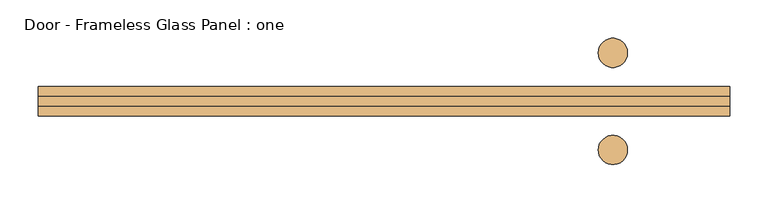
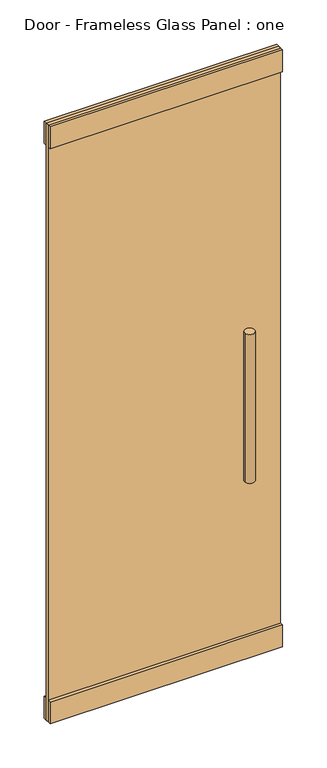
"""IFC4 building model written with IfcOpenShell, lengths in millimetres: door geometry, Door - Frameless Glass Panel : one."""

import ifcopenshell
import ifcopenshell.guid

model = None  # the IFC model being written
_history = None  # IfcOwnerHistory: only IFC2X3 demands one
_inside = {}  # id of a spatial element -> (the spatial element, [elements in it])
_under = {}  # id of a project, library or spatial element -> (it, [spatial elements below it])
_declared = {}  # id of a project -> (the project, [libraries it declares])
_typed = {}  # id of a type object -> (the type object, [elements of that type])
_made_of = {}  # id of a material, layer set ... -> (it, [elements and type objects made of it])


def new_model(schema):
    """Start an empty IFC model of exactly this schema.

    Asked for "IFC4X3", IfcOpenShell would pick the latest addendum, in which some entities
    have other attributes; the version numbers below select the first issue.
    IFC2X3 requires an IfcOwnerHistory on every rooted entity: one is made here for all.
    """
    global model, _history
    if schema == "IFC4X3":
        model = ifcopenshell.file(schema_version=(4, 3, 0, 0))
    else:
        model = ifcopenshell.file(schema=schema)
    _inside.clear()
    _under.clear()
    _declared.clear()
    _typed.clear()
    _made_of.clear()
    _history = None
    if model.schema == "IFC2X3":
        org = make("IfcOrganization", Name="unknown")
        user = make(
            "IfcPersonAndOrganization",
            ThePerson=make("IfcPerson", FamilyName="unknown"),
            TheOrganization=org,
        )
        app = make(
            "IfcApplication",
            ApplicationDeveloper=org,
            Version="unknown",
            ApplicationFullName="unknown",
            ApplicationIdentifier="unknown",
        )
        _history = make(
            "IfcOwnerHistory",
            OwningUser=user,
            OwningApplication=app,
            ChangeAction="ADDED",
            CreationDate=0,
        )
    return model


def make(cls, **values):
    """One entity of the class cls with the attributes given. An attribute that is None is left unset."""
    return model.create_entity(
        cls, **{name: value for name, value in values.items() if value is not None}
    )


def rooted(cls, **values):
    """An entity with a GlobalId (a new one), such as an element, a storey or a relation."""
    return make(cls, GlobalId=ifcopenshell.guid.new(), OwnerHistory=_history, **values)


def si_unit(unit_type, name, prefix=None):
    """IfcSIUnit, for example si_unit("LENGTHUNIT", "METRE", prefix="MILLI")."""
    return make("IfcSIUnit", UnitType=unit_type, Prefix=prefix, Name=name)


def assignment(units):
    """IfcUnitAssignment: the units of a project."""
    return None if units is None else make("IfcUnitAssignment", Units=units)


def point(xyz):
    """IfcCartesianPoint."""
    return None if xyz is None else make("IfcCartesianPoint", Coordinates=xyz)


def direction(xyz):
    """IfcDirection."""
    return None if xyz is None else make("IfcDirection", DirectionRatios=xyz)


def frame(location, z_axis=None, x_axis=None):
    """IfcAxis2Placement3D, a coordinate frame: its origin and axes. An axis left out is left unset."""
    return make(
        "IfcAxis2Placement3D",
        Location=point(location),
        Axis=direction(z_axis),
        RefDirection=direction(x_axis),
    )


def frame_2d(location, x_axis=None):
    """IfcAxis2Placement2D, a coordinate frame in the plane: its origin and x axis."""
    return make(
        "IfcAxis2Placement2D", Location=point(location), RefDirection=direction(x_axis)
    )


def origin():
    """The frame at (0, 0, 0) with its axes left unset."""
    return frame((0.0, 0.0, 0.0))


def origin_with_axes():
    """The frame at (0, 0, 0) with the z axis (0, 0, 1) and the x axis (1, 0, 0) written out."""
    return frame((0.0, 0.0, 0.0), z_axis=(0.0, 0.0, 1.0), x_axis=(1.0, 0.0, 0.0))


def place(relative_to, where):
    """IfcLocalPlacement: puts the frame where relative to a parent placement (None: the world)."""
    return make(
        "IfcLocalPlacement", PlacementRelTo=relative_to, RelativePlacement=where
    )


def context(
    kind, dimensions, precision=None, world=None, true_north=None, identifier=None
):
    """IfcGeometricRepresentationContext, for example the 3D "Model" context."""
    return make(
        "IfcGeometricRepresentationContext",
        ContextIdentifier=identifier,
        ContextType=kind,
        CoordinateSpaceDimension=dimensions,
        Precision=precision,
        WorldCoordinateSystem=world,
        TrueNorth=true_north,
    )


def project(units=None, contexts=None):
    """IfcProject with its units and contexts."""
    return rooted(
        "IfcProject",
        Name="project",
        RepresentationContexts=contexts,
        UnitsInContext=assignment(units),
    )


def spatial(cls, under=None, at=None, **own):
    """A site, building, storey or space (cls), placed at a placement, below another one or the project."""
    s = rooted(cls, ObjectPlacement=at, **own)
    if under is not None:
        _under.setdefault(under.id(), (under, []))[1].append(s)
    return s


def polyline(points):
    """IfcPolyline through the points."""
    return make("IfcPolyline", Points=[point(p) for p in points])


def circle_curve(where, radius):
    """IfcCircle in the frame where."""
    return make("IfcCircle", Position=where, Radius=radius)


def trimmed(basis, trim1, trim2, sense, master):
    """IfcTrimmedCurve: the piece of a basis curve between two trims."""
    return make(
        "IfcTrimmedCurve",
        BasisCurve=basis,
        Trim1=trim1,
        Trim2=trim2,
        SenseAgreement=sense,
        MasterRepresentation=master,
    )


def segment(curve, same_sense, transition):
    """IfcCompositeCurveSegment."""
    return make(
        "IfcCompositeCurveSegment",
        Transition=transition,
        SameSense=same_sense,
        ParentCurve=curve,
    )


def composite_curve(segments, self_intersect=None):
    """IfcCompositeCurve: segments joined end to end."""
    return make("IfcCompositeCurve", Segments=segments, SelfIntersect=self_intersect)


def outline(outer, holes=None, kind="AREA"):
    """IfcArbitraryClosedProfileDef: a profile drawn as a closed curve; with holes, ...WithVoids."""
    if holes is None:
        return make("IfcArbitraryClosedProfileDef", ProfileType=kind, OuterCurve=outer)
    return make(
        "IfcArbitraryProfileDefWithVoids",
        ProfileType=kind,
        OuterCurve=outer,
        InnerCurves=holes,
    )


def extrude(swept, where, along, depth):
    """IfcExtrudedAreaSolid: the profile swept, set in the frame where, extruded along a direction by depth."""
    return make(
        "IfcExtrudedAreaSolid",
        SweptArea=swept,
        Position=where,
        ExtrudedDirection=direction(along),
        Depth=depth,
    )


def shape(context_of_items, identifier, shape_type, items):
    """IfcShapeRepresentation: the items that make up one representation, for example the "Body"."""
    return make(
        "IfcShapeRepresentation",
        ContextOfItems=context_of_items,
        RepresentationIdentifier=identifier,
        RepresentationType=shape_type,
        Items=items,
    )


def source(mapping_origin, context_of_items, identifier, shape_type, items):
    """IfcRepresentationMap: a shape defined once, which mapped items show again and again."""
    return make(
        "IfcRepresentationMap",
        MappingOrigin=mapping_origin,
        MappedRepresentation=shape(context_of_items, identifier, shape_type, items),
    )


def transform(
    local_origin,
    x_axis=None,
    y_axis=None,
    z_axis=None,
    scale=None,
    scale2=None,
    scale3=None,
    uniform=True,
):
    """IfcCartesianTransformationOperator3D, or its non-uniform kind. x_axis, y_axis, z_axis: its Axis1, 2, 3."""
    if uniform:
        return make(
            "IfcCartesianTransformationOperator3D",
            Axis1=direction(x_axis),
            Axis2=direction(y_axis),
            LocalOrigin=point(local_origin),
            Scale=scale,
            Axis3=direction(z_axis),
        )
    return make(
        "IfcCartesianTransformationOperator3DnonUniform",
        Axis1=direction(x_axis),
        Axis2=direction(y_axis),
        LocalOrigin=point(local_origin),
        Scale=scale,
        Axis3=direction(z_axis),
        Scale2=scale2,
        Scale3=scale3,
    )


def mapped(mapping_source, mapping_target):
    """IfcMappedItem: shows the shape of a source again, moved by a transform."""
    return make(
        "IfcMappedItem", MappingSource=mapping_source, MappingTarget=mapping_target
    )


def made_of(thing, what):
    """Note that an element or type object is made of a material, layer set ...; save() writes the relation."""
    if what is not None:
        _made_of.setdefault(what.id(), (what, []))[1].append(thing)
    return thing


def element(
    cls,
    number,
    at=None,
    inside=None,
    cuts=None,
    type_object=None,
    material=None,
    context=None,
    identifier="Body",
    shape_type=None,
    held_by="IfcProductDefinitionShape",
    body=None,
    shapes=None,
    **own,
):
    """One element of the class cls, such as IfcWall. Its Tag is "e" and its number.

    at: its placement. inside: the storey or other place that contains it. cuts: it is an
    opening in that element (IfcRelVoidsElement). A single representation is given by context,
    identifier, shape_type and body (its items); several are given by shapes. held_by: the class
    of the entity that holds the representations. save() writes the other relations.
    """
    e = rooted(cls, Tag="e%d" % number, ObjectPlacement=at, **own)
    if body is not None:
        shapes = [shape(context, identifier, shape_type, body)]
    if shapes is not None:
        e.Representation = make(held_by, Representations=shapes)
    if inside is not None:
        _inside.setdefault(inside.id(), (inside, []))[1].append(e)
    if cuts is not None:
        rooted(
            "IfcRelVoidsElement", RelatingBuildingElement=cuts, RelatedOpeningElement=e
        )
    if type_object is not None:
        _typed.setdefault(type_object.id(), (type_object, []))[1].append(e)
    return made_of(e, material)


def aggregate(whole, parts):
    """IfcRelAggregates: a whole, such as a stair, and the parts it consists of."""
    return rooted("IfcRelAggregates", RelatingObject=whole, RelatedObjects=parts)


def save(model, path):
    """Write the relations noted so far, then the file.

    IfcRelAggregates (storeys below a building ...), IfcRelContainedInSpatialStructure (elements
    in a storey), IfcRelDefinesByType, IfcRelAssociatesMaterial and IfcRelDeclares: one each for
    every whole, place, type object, material and project.
    """
    for whole, parts in _under.values():
        aggregate(whole, parts)
    for where, things in _inside.values():
        rooted(
            "IfcRelContainedInSpatialStructure",
            RelatedElements=things,
            RelatingStructure=where,
        )
    for kind, things in _typed.values():
        rooted("IfcRelDefinesByType", RelatedObjects=things, RelatingType=kind)
    for what, things in _made_of.values():
        rooted("IfcRelAssociatesMaterial", RelatedObjects=things, RelatingMaterial=what)
    for by, libraries in _declared.values():
        rooted("IfcRelDeclares", RelatingContext=by, RelatedDefinitions=libraries)
    model.write(path)


def door_frameless_glass_panel_one_304fad4e(model_context):
    return source(origin(), model_context, "Body", "SweptSolid", [
        extrude(outline(composite_curve([segment(trimmed(circle_curve(frame_2d((298.45, -63.5)), 19.05), [point((279.4, -63.5))], [point((317.5, -63.5))], False, "CARTESIAN"), True, "CONTINUOUS"), segment(trimmed(circle_curve(frame_2d((298.45, -63.5)), 19.05), [point((317.5, -63.5))], [point((279.4, -63.5))], False, "CARTESIAN"), True, "CONTINUOUS")], self_intersect=False)), frame((0.0, 0.0, 762.0), z_axis=(0.0, 0.0, 1.0), x_axis=(1.0, 0.0, 0.0)), (0.0, 0.0, 1.0), 609.6),
        extrude(outline(composite_curve([segment(trimmed(circle_curve(frame_2d((298.45, 63.5)), 19.05), [point((279.4, 63.5))], [point((317.5, 63.5))], False, "CARTESIAN"), True, "CONTINUOUS"), segment(trimmed(circle_curve(frame_2d((298.45, 63.5)), 19.05), [point((317.5, 63.5))], [point((279.4, 63.5))], False, "CARTESIAN"), True, "CONTINUOUS")], self_intersect=False)), frame((0.0, 0.0, 762.0), z_axis=(0.0, 0.0, 1.0), x_axis=(1.0, 0.0, 0.0)), (0.0, 0.0, 1.0), 609.6),
        extrude(outline(polyline([(450.85, 6.35), (450.85, -6.35), (-450.85, -6.35), (-450.85, 6.35), (450.85, 6.35)])), origin_with_axes(), (0.0, 0.0, 1.0), 2444.75),
        extrude(outline(polyline([(-450.85, 19.05), (450.85, 19.05), (450.85, -19.05), (-450.85, -19.05), (-450.85, 19.05)])), origin_with_axes(), (0.0, 0.0, 1.0), 88.9),
        extrude(outline(polyline([(-450.85, 19.05), (450.85, 19.05), (450.85, -19.05), (-450.85, -19.05), (-450.85, 19.05)])), frame((0.0, 0.0, 2355.85), z_axis=(0.0, 0.0, 1.0), x_axis=(1.0, 0.0, 0.0)), (0.0, 0.0, 1.0), 88.9),
    ])


if __name__ == "__main__":
    model = new_model("IFC4")
    model_context = context("Model", 3, world=origin())
    ifc_project = project(units=[si_unit("LENGTHUNIT", "METRE", prefix="MILLI")], contexts=[model_context])
    site = spatial("IfcSite", under=ifc_project)
    building = spatial("IfcBuilding", under=site)
    placement = place(None, origin())
    door_frameless_glass_panel_one_shape = door_frameless_glass_panel_one_304fad4e(model_context)
    element("IfcDoor", 1, ObjectType="Door - Frameless Glass Panel : one", at=placement, inside=building, context=model_context, shape_type="MappedRepresentation", body=[
        mapped(door_frameless_glass_panel_one_shape, transform((0.0, 0.0, 0.0), x_axis=(1.0, 0.0, 0.0), y_axis=(0.0, 1.0, 0.0), z_axis=(0.0, 0.0, 1.0))),
    ])
    save(model, "model.ifc")

# Revit data of these elements
# Type "Door - Frameless Glass Panel : one"
#   Type Mark = "8"
#   Analytic Construction = "<None>"
#   Pivot Point [instance default] = 5' - 2.25212"
#   Glass Thickness = 0' - 0 1/2"
#   Gap btwn Panels = 0' - 0 1/4"
#   Panel Material = CLEAR TEMPERED GLASS (HEAD/SILL SUPPORT DETAILS TO MATCHING EXISTING FRAMLESS GLASS DETAILS @ TENANT ENTRANCE)
#   Handle Material = ALUM
# Element 1 (IfcDoor, "Door - Frameless Glass Panel : one")
#   Materials on its faces: "ALUM", "CLEAR TEMPERED GLASS (HEAD/SILL SUPPORT DETAILS TO MATCHING EXISTING FRAMLESS GLASS DETAILS @ TENANT ENTRANCE)"
# Materials
#   "CLEAR TEMPERED GLASS (HEAD/SILL SUPPORT DETAILS TO MATCHING EXISTING FRAMLESS GLASS DETAILS @ TENANT ENTRANCE)": class "Glass", colour RGB 218 227 224, transparency 1, Description = "Soda Lime Glass", Cost = 0
#   "ALUM": class "Generic", colour RGB 157 157 157, transparency 0, Cost = 0
